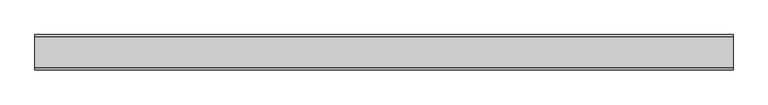
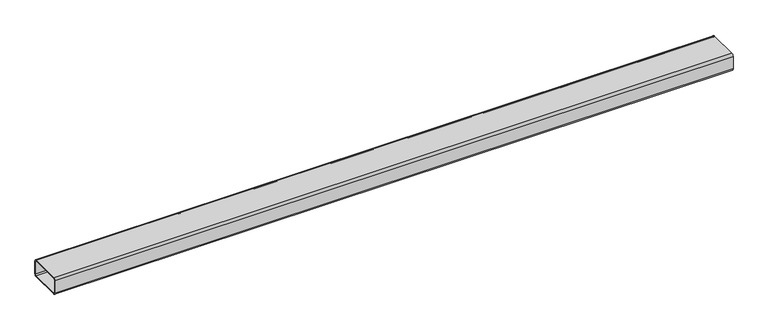
"""IFC4 building model written with IfcOpenShell, lengths in millimetres: proxy geometry, Louvre frame001 295 : Louvre frame001 295."""

from ifc_helpers import new_model, si_unit, point, frame, frame_2d, origin, place, context, project, spatial, polyline, circle_curve, trimmed, segment, composite_curve, outline, extrude, source, transform, mapped, element, save


def generic_models_43cd0ce6(model_context):
    return source(origin(), model_context, "Body", "SweptSolid", [
        extrude(outline(composite_curve([segment(trimmed(circle_curve(frame_2d((9795.5719584, 37502.846)), 6.35), [point((9795.5719584, 37496.496))], [point((9789.2219584, 37502.846))], False, "CARTESIAN"), True, "CONTINUOUS"), segment(polyline([(9789.2219584, 37502.846), (9789.2219584, 37540.946)]), True, "CONTINUOUS"), segment(trimmed(circle_curve(frame_2d((9795.5719584, 37540.946)), 6.35), [point((9789.2219584, 37540.946))], [point((9795.5719584, 37547.296))], False, "CARTESIAN"), True, "CONTINUOUS"), segment(polyline([(9795.5719584, 37547.296), (9884.4719584, 37547.296)]), True, "CONTINUOUS"), segment(trimmed(circle_curve(frame_2d((9884.4719584, 37540.946)), 6.35), [point((9884.4719584, 37547.296))], [point((9890.8219584, 37540.946))], False, "CARTESIAN"), True, "CONTINUOUS"), segment(polyline([(9890.8219584, 37540.946), (9890.8219584, 37502.846)]), True, "CONTINUOUS"), segment(trimmed(circle_curve(frame_2d((9884.4719584, 37502.846)), 6.35), [point((9890.8219584, 37502.846))], [point((9884.4719584, 37496.496))], False, "CARTESIAN"), True, "CONTINUOUS"), segment(polyline([(9884.4719584, 37496.496), (9795.5719584, 37496.496)]), True, "CONTINUOUS")], self_intersect=False), holes=[composite_curve([segment(polyline([(9887.6519584, 37502.846), (9887.6519584, 37540.946)]), True, "CONTINUOUS"), segment(trimmed(circle_curve(frame_2d((9884.4719584, 37540.946)), 3.18), [point((9887.6519584, 37540.946))], [point((9884.4719584, 37544.126))], True, "CARTESIAN"), True, "CONTINUOUS"), segment(polyline([(9884.4719584, 37544.126), (9795.5719584, 37544.126)]), True, "CONTINUOUS"), segment(trimmed(circle_curve(frame_2d((9795.5719584, 37540.946)), 3.18), [point((9795.5719584, 37544.126))], [point((9792.3919584, 37540.946))], True, "CARTESIAN"), True, "CONTINUOUS"), segment(polyline([(9792.3919584, 37540.946), (9792.3919584, 37502.846)]), True, "CONTINUOUS"), segment(trimmed(circle_curve(frame_2d((9795.5719584, 37502.846)), 3.18), [point((9792.3919584, 37502.846))], [point((9795.5719584, 37499.666))], True, "CARTESIAN"), True, "CONTINUOUS"), segment(polyline([(9795.5719584, 37499.666), (9884.4719584, 37499.666)]), True, "CONTINUOUS"), segment(trimmed(circle_curve(frame_2d((9884.4719584, 37502.846)), 3.18), [point((9884.4719584, 37499.666))], [point((9887.6519584, 37502.846))], True, "CARTESIAN"), True, "CONTINUOUS")], self_intersect=False)]), frame((3694.2883192, 0.0, 0.0), z_axis=(1.0, 0.0, 0.0), x_axis=(0.0, 1.0, 0.0)), (0.0, 0.0, 1.0), 2000.0),
    ])


if __name__ == "__main__":
    model = new_model("IFC4")
    model_context = context("Model", 3, world=origin())
    ifc_project = project(units=[si_unit("LENGTHUNIT", "METRE", prefix="MILLI")], contexts=[model_context])
    site = spatial("IfcSite", under=ifc_project)
    building = spatial("IfcBuilding", under=site)
    placement = place(None, origin())
    generic_models_shape = generic_models_43cd0ce6(model_context)
    element("IfcBuildingElementProxy", 1, Name="Louvre frame001 295 : Louvre frame001 295", ObjectType="Louvre frame001 295 : Louvre frame001 295", at=placement, inside=building, context=model_context, shape_type="MappedRepresentation", body=[
        mapped(generic_models_shape, transform((0.0, 0.0, 0.0), x_axis=(1.0, 0.0, 0.0), y_axis=(0.0, 1.0, 0.0), z_axis=(0.0, 0.0, 1.0))),
    ])
    save(model, "model.ifc")

# Revit data of these elements
# Type "Louvre frame001 295 : Louvre frame001 295"
#   NameOverride = "Louvre frame001"
# Element 1 (IfcBuildingElementProxy, "Louvre frame001 295 : Louvre frame001 295")
#   Materials on its faces: "ALUMINIUM LOUVRE - TBD"
# Materials
#   "ALUMINIUM LOUVRE - TBD": class "Unassigned", colour RGB 92 107 122, transparency 0
